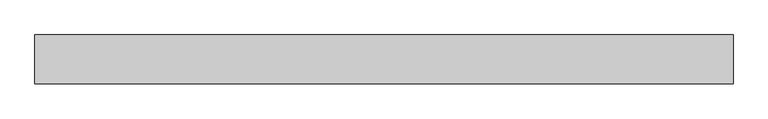
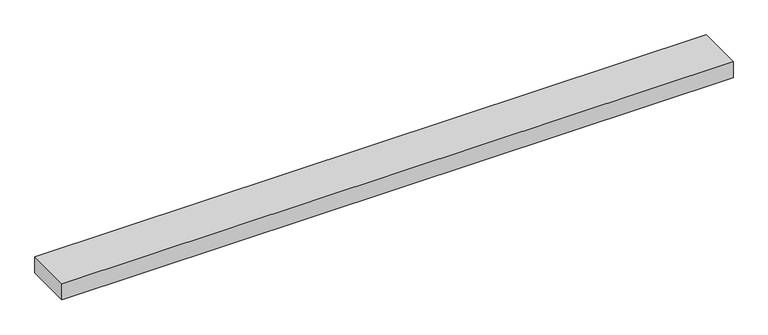
"""IFC4 building model written with IfcOpenShell, lengths in millimetres: proxy geometry, Blocking010 1441 : Blocking010 1441."""

import ifcopenshell
import ifcopenshell.guid

model = None  # the IFC model being written
_history = None  # IfcOwnerHistory: only IFC2X3 demands one
_inside = {}  # id of a spatial element -> (the spatial element, [elements in it])
_under = {}  # id of a project, library or spatial element -> (it, [spatial elements below it])
_declared = {}  # id of a project -> (the project, [libraries it declares])
_typed = {}  # id of a type object -> (the type object, [elements of that type])
_made_of = {}  # id of a material, layer set ... -> (it, [elements and type objects made of it])


def new_model(schema):
    """Start an empty IFC model of exactly this schema.

    Asked for "IFC4X3", IfcOpenShell would pick the latest addendum, in which some entities
    have other attributes; the version numbers below select the first issue.
    IFC2X3 requires an IfcOwnerHistory on every rooted entity: one is made here for all.
    """
    global model, _history
    if schema == "IFC4X3":
        model = ifcopenshell.file(schema_version=(4, 3, 0, 0))
    else:
        model = ifcopenshell.file(schema=schema)
    _inside.clear()
    _under.clear()
    _declared.clear()
    _typed.clear()
    _made_of.clear()
    _history = None
    if model.schema == "IFC2X3":
        org = make("IfcOrganization", Name="unknown")
        user = make(
            "IfcPersonAndOrganization",
            ThePerson=make("IfcPerson", FamilyName="unknown"),
            TheOrganization=org,
        )
        app = make(
            "IfcApplication",
            ApplicationDeveloper=org,
            Version="unknown",
            ApplicationFullName="unknown",
            ApplicationIdentifier="unknown",
        )
        _history = make(
            "IfcOwnerHistory",
            OwningUser=user,
            OwningApplication=app,
            ChangeAction="ADDED",
            CreationDate=0,
        )
    return model


def make(cls, **values):
    """One entity of the class cls with the attributes given. An attribute that is None is left unset."""
    return model.create_entity(
        cls, **{name: value for name, value in values.items() if value is not None}
    )


def rooted(cls, **values):
    """An entity with a GlobalId (a new one), such as an element, a storey or a relation."""
    return make(cls, GlobalId=ifcopenshell.guid.new(), OwnerHistory=_history, **values)


def si_unit(unit_type, name, prefix=None):
    """IfcSIUnit, for example si_unit("LENGTHUNIT", "METRE", prefix="MILLI")."""
    return make("IfcSIUnit", UnitType=unit_type, Prefix=prefix, Name=name)


def assignment(units):
    """IfcUnitAssignment: the units of a project."""
    return None if units is None else make("IfcUnitAssignment", Units=units)


def point(xyz):
    """IfcCartesianPoint."""
    return None if xyz is None else make("IfcCartesianPoint", Coordinates=xyz)


def direction(xyz):
    """IfcDirection."""
    return None if xyz is None else make("IfcDirection", DirectionRatios=xyz)


def frame(location, z_axis=None, x_axis=None):
    """IfcAxis2Placement3D, a coordinate frame: its origin and axes. An axis left out is left unset."""
    return make(
        "IfcAxis2Placement3D",
        Location=point(location),
        Axis=direction(z_axis),
        RefDirection=direction(x_axis),
    )


def origin():
    """The frame at (0, 0, 0) with its axes left unset."""
    return frame((0.0, 0.0, 0.0))


def place(relative_to, where):
    """IfcLocalPlacement: puts the frame where relative to a parent placement (None: the world)."""
    return make(
        "IfcLocalPlacement", PlacementRelTo=relative_to, RelativePlacement=where
    )


def context(
    kind, dimensions, precision=None, world=None, true_north=None, identifier=None
):
    """IfcGeometricRepresentationContext, for example the 3D "Model" context."""
    return make(
        "IfcGeometricRepresentationContext",
        ContextIdentifier=identifier,
        ContextType=kind,
        CoordinateSpaceDimension=dimensions,
        Precision=precision,
        WorldCoordinateSystem=world,
        TrueNorth=true_north,
    )


def project(units=None, contexts=None):
    """IfcProject with its units and contexts."""
    return rooted(
        "IfcProject",
        Name="project",
        RepresentationContexts=contexts,
        UnitsInContext=assignment(units),
    )


def spatial(cls, under=None, at=None, **own):
    """A site, building, storey or space (cls), placed at a placement, below another one or the project."""
    s = rooted(cls, ObjectPlacement=at, **own)
    if under is not None:
        _under.setdefault(under.id(), (under, []))[1].append(s)
    return s


def polyline(points):
    """IfcPolyline through the points."""
    return make("IfcPolyline", Points=[point(p) for p in points])


def outline(outer, holes=None, kind="AREA"):
    """IfcArbitraryClosedProfileDef: a profile drawn as a closed curve; with holes, ...WithVoids."""
    if holes is None:
        return make("IfcArbitraryClosedProfileDef", ProfileType=kind, OuterCurve=outer)
    return make(
        "IfcArbitraryProfileDefWithVoids",
        ProfileType=kind,
        OuterCurve=outer,
        InnerCurves=holes,
    )


def extrude(swept, where, along, depth):
    """IfcExtrudedAreaSolid: the profile swept, set in the frame where, extruded along a direction by depth."""
    return make(
        "IfcExtrudedAreaSolid",
        SweptArea=swept,
        Position=where,
        ExtrudedDirection=direction(along),
        Depth=depth,
    )


def shape(context_of_items, identifier, shape_type, items):
    """IfcShapeRepresentation: the items that make up one representation, for example the "Body"."""
    return make(
        "IfcShapeRepresentation",
        ContextOfItems=context_of_items,
        RepresentationIdentifier=identifier,
        RepresentationType=shape_type,
        Items=items,
    )


def source(mapping_origin, context_of_items, identifier, shape_type, items):
    """IfcRepresentationMap: a shape defined once, which mapped items show again and again."""
    return make(
        "IfcRepresentationMap",
        MappingOrigin=mapping_origin,
        MappedRepresentation=shape(context_of_items, identifier, shape_type, items),
    )


def transform(
    local_origin,
    x_axis=None,
    y_axis=None,
    z_axis=None,
    scale=None,
    scale2=None,
    scale3=None,
    uniform=True,
):
    """IfcCartesianTransformationOperator3D, or its non-uniform kind. x_axis, y_axis, z_axis: its Axis1, 2, 3."""
    if uniform:
        return make(
            "IfcCartesianTransformationOperator3D",
            Axis1=direction(x_axis),
            Axis2=direction(y_axis),
            LocalOrigin=point(local_origin),
            Scale=scale,
            Axis3=direction(z_axis),
        )
    return make(
        "IfcCartesianTransformationOperator3DnonUniform",
        Axis1=direction(x_axis),
        Axis2=direction(y_axis),
        LocalOrigin=point(local_origin),
        Scale=scale,
        Axis3=direction(z_axis),
        Scale2=scale2,
        Scale3=scale3,
    )


def mapped(mapping_source, mapping_target):
    """IfcMappedItem: shows the shape of a source again, moved by a transform."""
    return make(
        "IfcMappedItem", MappingSource=mapping_source, MappingTarget=mapping_target
    )


def made_of(thing, what):
    """Note that an element or type object is made of a material, layer set ...; save() writes the relation."""
    if what is not None:
        _made_of.setdefault(what.id(), (what, []))[1].append(thing)
    return thing


def element(
    cls,
    number,
    at=None,
    inside=None,
    cuts=None,
    type_object=None,
    material=None,
    context=None,
    identifier="Body",
    shape_type=None,
    held_by="IfcProductDefinitionShape",
    body=None,
    shapes=None,
    **own,
):
    """One element of the class cls, such as IfcWall. Its Tag is "e" and its number.

    at: its placement. inside: the storey or other place that contains it. cuts: it is an
    opening in that element (IfcRelVoidsElement). A single representation is given by context,
    identifier, shape_type and body (its items); several are given by shapes. held_by: the class
    of the entity that holds the representations. save() writes the other relations.
    """
    e = rooted(cls, Tag="e%d" % number, ObjectPlacement=at, **own)
    if body is not None:
        shapes = [shape(context, identifier, shape_type, body)]
    if shapes is not None:
        e.Representation = make(held_by, Representations=shapes)
    if inside is not None:
        _inside.setdefault(inside.id(), (inside, []))[1].append(e)
    if cuts is not None:
        rooted(
            "IfcRelVoidsElement", RelatingBuildingElement=cuts, RelatedOpeningElement=e
        )
    if type_object is not None:
        _typed.setdefault(type_object.id(), (type_object, []))[1].append(e)
    return made_of(e, material)


def aggregate(whole, parts):
    """IfcRelAggregates: a whole, such as a stair, and the parts it consists of."""
    return rooted("IfcRelAggregates", RelatingObject=whole, RelatedObjects=parts)


def save(model, path):
    """Write the relations noted so far, then the file.

    IfcRelAggregates (storeys below a building ...), IfcRelContainedInSpatialStructure (elements
    in a storey), IfcRelDefinesByType, IfcRelAssociatesMaterial and IfcRelDeclares: one each for
    every whole, place, type object, material and project.
    """
    for whole, parts in _under.values():
        aggregate(whole, parts)
    for where, things in _inside.values():
        rooted(
            "IfcRelContainedInSpatialStructure",
            RelatedElements=things,
            RelatingStructure=where,
        )
    for kind, things in _typed.values():
        rooted("IfcRelDefinesByType", RelatedObjects=things, RelatingType=kind)
    for what, things in _made_of.values():
        rooted("IfcRelAssociatesMaterial", RelatedObjects=things, RelatingMaterial=what)
    for by, libraries in _declared.values():
        rooted("IfcRelDeclares", RelatingContext=by, RelatedDefinitions=libraries)
    model.write(path)


def generic_models_19c299ce(model_context):
    return source(origin(), model_context, "Body", "SweptSolid", [
        extrude(outline(polyline([(3694.2883192, 9590.6375834), (3694.2883192, 9730.3375834), (5694.2883192, 9730.3375834), (5694.2883192, 9590.6375834), (3694.2883192, 9590.6375834)])), frame((0.0, 0.0, 36531.296), z_axis=(0.0, 0.0, 1.0), x_axis=(1.0, 0.0, 0.0)), (0.0, 0.0, 1.0), 50.8),
    ])


if __name__ == "__main__":
    model = new_model("IFC4")
    model_context = context("Model", 3, world=origin())
    ifc_project = project(units=[si_unit("LENGTHUNIT", "METRE", prefix="MILLI")], contexts=[model_context])
    site = spatial("IfcSite", under=ifc_project)
    building = spatial("IfcBuilding", under=site)
    placement = place(None, origin())
    generic_models_shape = generic_models_19c299ce(model_context)
    element("IfcBuildingElementProxy", 1, Name="Blocking010 1441 : Blocking010 1441", ObjectType="Blocking010 1441 : Blocking010 1441", at=placement, inside=building, context=model_context, shape_type="MappedRepresentation", body=[
        mapped(generic_models_shape, transform((0.0, 0.0, 0.0), x_axis=(1.0, 0.0, 0.0), y_axis=(0.0, 1.0, 0.0), z_axis=(0.0, 0.0, 1.0))),
    ])
    save(model, "model.ifc")

# Revit data of these elements
# Type "Blocking010 1441 : Blocking010 1441"
#   NameOverride = "Blocking010"
# Element 1 (IfcBuildingElementProxy, "Blocking010 1441 : Blocking010 1441")
#   Materials on its faces: "WOOD BLOCKING AS REQUIRED"
# Materials
#   "WOOD BLOCKING AS REQUIRED": class "Unassigned", colour RGB 166 124 85, transparency 0, Cost = 0
